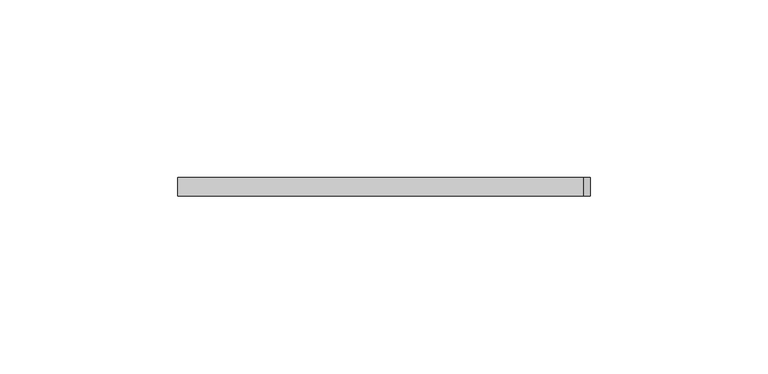
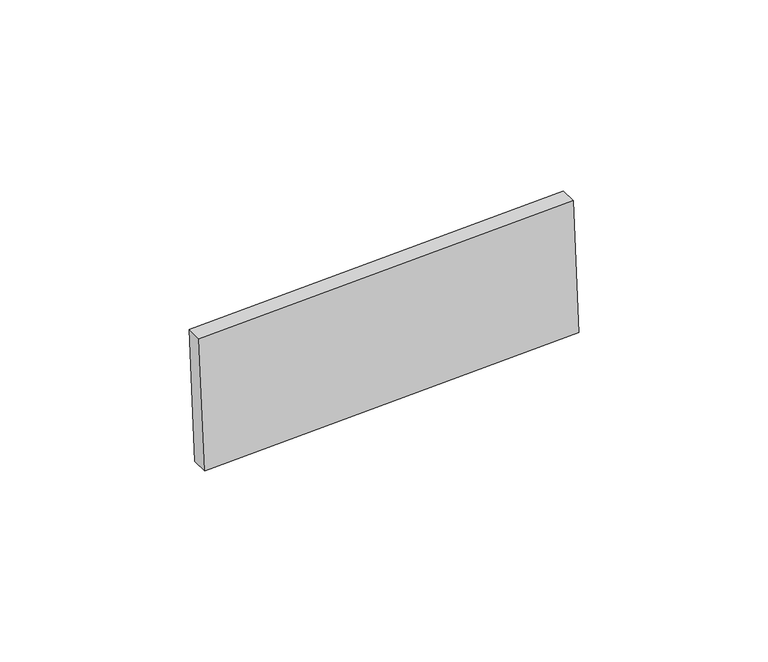
"""IFC4 building model written with IfcOpenShell, lengths in millimetres: proxy geometry, Inner panel:Inner panel:1:Inner panel:1 : Inner panel:Inner panel:300324:2:Inner panel:1:Inner panel:1 : Inner panel:Inner panel:300324:2 : Inner panel:Inner panel:1:Inner panel:1 : Inner panel:Inner panel:300324:300043:167 : Inner panel:Inner panel:1:Inner panel:1 : Inner panel:Inner panel:300324:2:Inner panel:1:Inner panel:1 : Inner panel:Inner panel:300324:2 : Inner panel:Inner panel:1:Inner panel:1 : Inner panel:Inner panel:300324:300043:308120."""

from ifc_helpers import new_model, si_unit, frame, origin, place, context, project, spatial, polyline, outline, extrude, source, transform, mapped, element, save


def generic_models_6c29cc45(model_context):
    return source(origin(), model_context, "Body", "SweptSolid", [
        extrude(outline(polyline([(0.0, -114.3), (0.0, 0.0), (5.213809, 0.0), (5.213809, -114.3), (0.0, -114.3)])), frame((560425.2415304, -565400.507991, 3954.8593665), z_axis=(-0.04163054471216399, 0.0, 0.9991330730923527), x_axis=(0.0, -1.0, 0.0)), (0.0, 0.0, 1.0), 43.2233908),
    ])


if __name__ == "__main__":
    model = new_model("IFC4")
    model_context = context("Model", 3, world=origin())
    ifc_project = project(units=[si_unit("LENGTHUNIT", "METRE", prefix="MILLI")], contexts=[model_context])
    site = spatial("IfcSite", under=ifc_project)
    building = spatial("IfcBuilding", under=site)
    placement = place(None, origin())
    generic_models_shape = generic_models_6c29cc45(model_context)
    element("IfcBuildingElementProxy", 1, Name="Inner panel:Inner panel:1:Inner panel:1 : Inner panel:Inner panel:300324:2:Inner panel:1:Inner panel:1 : Inner panel:Inner panel:300324:2 : Inner panel:Inner panel:1:Inner panel:1 : Inner panel:Inner panel:300324:300043:167 : Inner panel:Inner panel:1:Inner panel:1 : Inner panel:Inner panel:300324:2:Inner panel:1:Inner panel:1 : Inner panel:Inner panel:300324:2 : Inner panel:Inner panel:1:Inner panel:1 : Inner panel:Inner panel:300324:300043:308120", ObjectType="Inner panel:Inner panel:1:Inner panel:1 : Inner panel:Inner panel:300324:2:Inner panel:1:Inner panel:1 : Inner panel:Inner panel:300324:2 : Inner panel:Inner panel:1:Inner panel:1 : Inner panel:Inner panel:300324:300043:167 : Inner panel:Inner panel:1:Inner panel:1 : Inner panel:Inner panel:300324:2:Inner panel:1:Inner panel:1 : Inner panel:Inner panel:300324:2 : Inner panel:Inner panel:1:Inner panel:1 : Inner panel:Inner panel:300324:300043:308120", at=placement, inside=building, context=model_context, shape_type="MappedRepresentation", body=[
        mapped(generic_models_shape, transform((0.0, 0.0, 0.0), x_axis=(1.0, 0.0, 0.0), y_axis=(0.0, 1.0, 0.0), z_axis=(0.0, 0.0, 1.0))),
    ])
    save(model, "model.ifc")

# Revit data of these elements
# Type "Inner panel:Inner panel:1:Inner panel:1 : Inner panel:Inner panel:300324:2:Inner panel:1:Inner panel:1 : Inner panel:Inner panel:300324:2 : Inner panel:Inner panel:1:Inner panel:1 : Inner panel:Inner panel:300324:300043:167 : Inner panel:Inner panel:1:Inner panel:1 : Inner panel:Inner panel:300324:2:Inner panel:1:Inner panel:1 : Inner panel:Inner panel:300324:2 : Inner panel:Inner panel:1:Inner panel:1 : Inner panel:Inner panel:300324:300043:308120"
#   NameOverride = "Inner panel:Inner panel:1:Inner panel:1 : Inner panel:Inner panel:300324:2:Inner panel:1:Inner panel:1 : Inner panel:Inner panel:300324:2 : Inner panel:Inner panel:1:Inner panel:1 : Inner panel:Inner panel:300324:300043:308120"
#   ObjectTypeOverride = "Inner panel:1:Inner panel:1 : Inner panel:Inner panel:300324:2 : Inner panel:Inner panel:1:Inner panel:1 : Inner panel:Inner panel:300324:300043"
#   Reference = "Inner panel"
#   Tag = "308120"
# Element 1 (IfcBuildingElementProxy, "Inner panel:Inner panel:1:Inner panel:1 : Inner panel:Inner panel:300324:2:Inner panel:1:Inner panel:1 : Inner panel:Inner panel:300324:2 : Inner panel:Inner panel:1:Inner panel:1 : Inner panel:Inner panel:300324:300043:167 : Inner panel:Inner panel:1:Inner panel:1 : Inner panel:Inner panel:300324:2:Inner panel:1:Inner panel:1 : Inner panel:Inner panel:300324:2 : Inner panel:Inner panel:1:Inner panel:1 : Inner panel:Inner panel:300324:300043:308120")
#   Materials on its faces: "SLIDING CLIP"
# Materials
#   "SLIDING CLIP": class "Generic", colour RGB 120 120 120, transparency 0, Cost = 0
